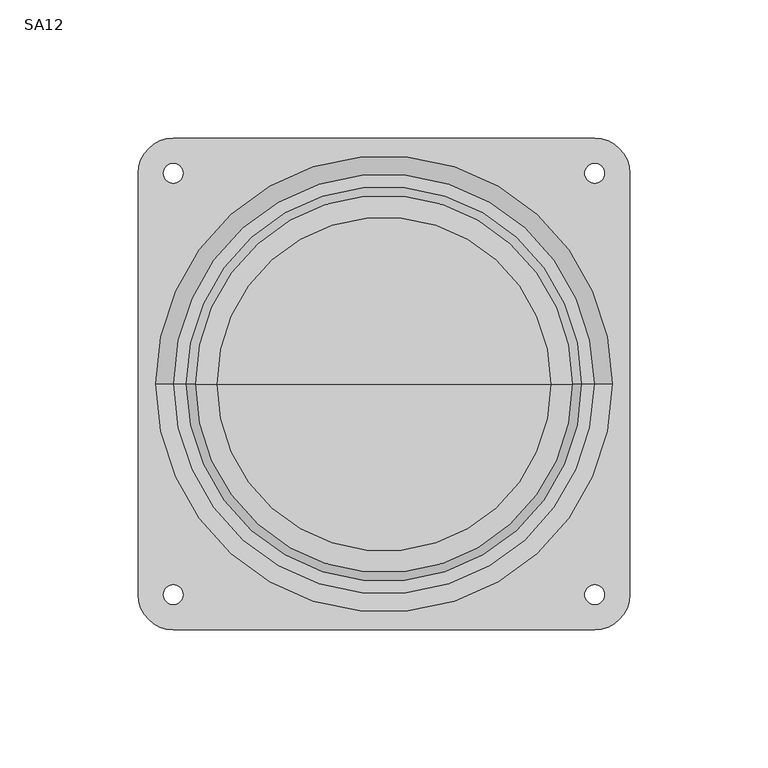
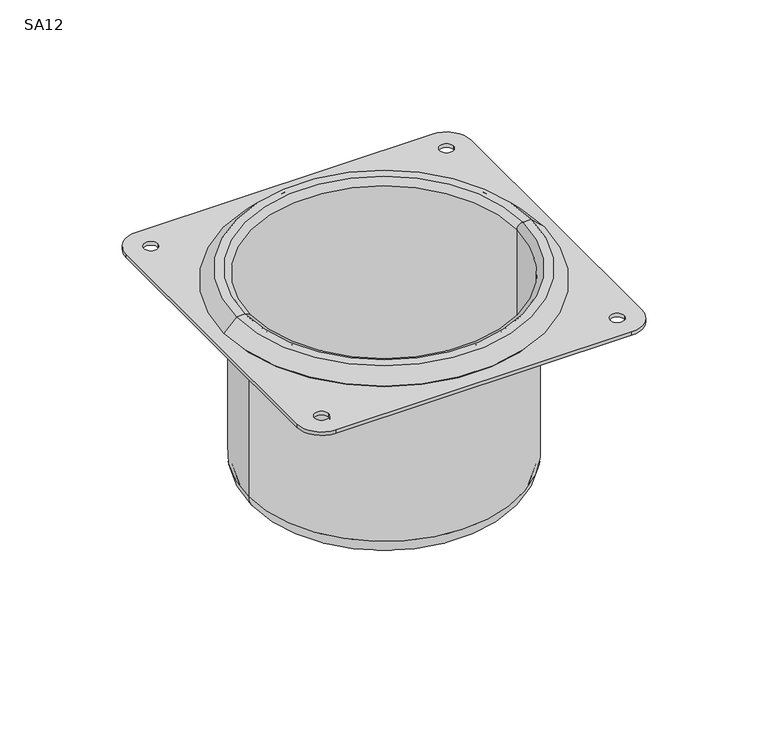
"""IFC4 building model written with IfcOpenShell, lengths in millimetres: proxy geometry, Security_Accessories-Bradley-SA12 : SA12."""

from ifc_helpers import new_model, si_unit, point, frame, frame_2d, origin, origin_with_axes, origin_2d, place, context, project, spatial, polyline, circle_curve, ellipse_curve, trimmed, segment, composite_curve, outline, extrude, source, transform, mapped, element, save
from ifc_brep_helpers import plane_surface, cylinder_surface, revolved_surface, advanced_brep


def sa12_a1c1abd2(model_context):
    return source(origin(), model_context, "Body", "SolidModel", [
        extrude(outline(composite_curve([segment(trimmed(circle_curve(frame_2d((-76.2, 76.2)), 12.7), [point((-88.9, 76.2))], [point((-76.2, 88.9))], False, "CARTESIAN"), True, "CONTINUOUS"), segment(polyline([(-76.2, 88.9), (76.2, 88.9)]), True, "CONTINUOUS"), segment(trimmed(circle_curve(frame_2d((76.2, 76.2)), 12.7), [point((76.2, 88.9))], [point((88.9, 76.2))], False, "CARTESIAN"), True, "CONTINUOUS"), segment(polyline([(88.9, 76.2), (88.9, -76.2)]), True, "CONTINUOUS"), segment(trimmed(circle_curve(frame_2d((76.2, -76.2)), 12.7), [point((88.9, -76.2))], [point((76.2, -88.9))], False, "CARTESIAN"), True, "CONTINUOUS"), segment(polyline([(76.2, -88.9), (-76.2, -88.9)]), True, "CONTINUOUS"), segment(trimmed(circle_curve(frame_2d((-76.2, -76.2)), 12.7), [point((-76.2, -88.9))], [point((-88.9, -76.2))], False, "CARTESIAN"), True, "CONTINUOUS"), segment(polyline([(-88.9, -76.2), (-88.9, 76.2)]), True, "CONTINUOUS")], self_intersect=False), holes=[composite_curve([segment(trimmed(circle_curve(frame_2d((-76.2, 76.2)), 3.571875), [point((-79.771875, 76.2))], [point((-72.628125, 76.2))], True, "CARTESIAN"), True, "CONTINUOUS"), segment(trimmed(circle_curve(frame_2d((-76.2, 76.2)), 3.571875), [point((-72.628125, 76.2))], [point((-79.771875, 76.2))], True, "CARTESIAN"), True, "CONTINUOUS")], self_intersect=False), composite_curve([segment(trimmed(circle_curve(frame_2d((-76.2, -76.2)), 3.571875), [point((-79.771875, -76.2))], [point((-72.628125, -76.2))], True, "CARTESIAN"), True, "CONTINUOUS"), segment(trimmed(circle_curve(frame_2d((-76.2, -76.2)), 3.571875), [point((-72.628125, -76.2))], [point((-79.771875, -76.2))], True, "CARTESIAN"), True, "CONTINUOUS")], self_intersect=False), composite_curve([segment(trimmed(circle_curve(frame_2d((76.2, -76.2)), 3.571875), [point((72.628125, -76.2))], [point((79.771875, -76.2))], True, "CARTESIAN"), True, "CONTINUOUS"), segment(trimmed(circle_curve(frame_2d((76.2, -76.2)), 3.571875), [point((79.771875, -76.2))], [point((72.628125, -76.2))], True, "CARTESIAN"), True, "CONTINUOUS")], self_intersect=False), composite_curve([segment(trimmed(circle_curve(frame_2d((76.2, 76.2)), 3.571875), [point((72.628125, 76.2))], [point((79.771875, 76.2))], True, "CARTESIAN"), True, "CONTINUOUS"), segment(trimmed(circle_curve(frame_2d((76.2, 76.2)), 3.571875), [point((79.771875, 76.2))], [point((72.628125, 76.2))], True, "CARTESIAN"), True, "CONTINUOUS")], self_intersect=False), composite_curve([segment(trimmed(circle_curve(origin_2d(), 81.4723693), [point((-81.4723693, 0.0))], [point((81.4723693, 0.0))], True, "CARTESIAN"), True, "CONTINUOUS"), segment(trimmed(circle_curve(origin_2d(), 81.4723693), [point((81.4723693, 0.0))], [point((-81.4723693, 0.0))], True, "CARTESIAN"), True, "CONTINUOUS")], self_intersect=False)]), origin_with_axes(), (0.0, 0.0, 1.0), 1.905),
        advanced_brep(
        [(68.326, 0.0, 6.4135), (-68.326, 0.0, 6.4135), (-68.326, 0.0, -90.551), (68.326, 0.0, -90.551), (71.4375, 0.0, 9.525), (-71.4375, 0.0, 9.525), (76.0076307, 0.0, 9.525), (-76.0076307, 0.0, 9.525), (82.55, 0.0, 2.9826307), (-82.55, 0.0, 2.9826307), (81.4723693, 0.0, 1.905), (-81.4723693, 0.0, 1.905), (75.3763693, 0.0, 8.001), (-75.3763693, 0.0, 8.001), (71.4375, 0.0, 8.001), (-71.4375, 0.0, 8.001), (69.85, 0.0, 6.4135), (-69.85, 0.0, 6.4135), (69.85, 0.0, -90.551), (-69.85, 0.0, -90.551), (60.3885, 0.0, -100.0125), (-60.3885, 0.0, -100.0125), (0.0, 0.0, -100.0125), (60.3885, 0.0, -98.4885), (-60.3885, 0.0, -98.4885), (0.0, 0.0, -98.4885)],
        [
            (0, 1, circle_curve(frame((0.0, 0.0, 6.4135), z_axis=(0.0, 0.0, 1.0), x_axis=(-1.0, 0.0, 0.0)), 68.326)),
            (1, 2),
            (2, 3, circle_curve(frame((0.0, 0.0, -90.551), z_axis=(0.0, 0.0, -1.0), x_axis=(-1.0, 0.0, 0.0)), 68.326)),
            (3, 0),
            (1, 0, circle_curve(frame((0.0, 0.0, 6.4135), z_axis=(0.0, 0.0, 1.0), x_axis=(-1.0, 0.0, 0.0)), 68.326)),
            (3, 2, circle_curve(frame((0.0, 0.0, -90.551), z_axis=(0.0, 0.0, -1.0), x_axis=(-1.0, 0.0, 0.0)), 68.326)),
            (4, 5, circle_curve(frame((0.0, 0.0, 9.525), z_axis=(0.0, 0.0, 1.0), x_axis=(-1.0, 0.0, 0.0)), 71.4375)),
            (5, 1, circle_curve(frame((-71.4375, 0.0, 6.4135), z_axis=(0.0, 1.0, 0.0), x_axis=(1.0, 0.0, 0.0)), 3.1115)),
            (0, 4, circle_curve(frame((71.4375, 0.0, 6.4135), z_axis=(0.0, 1.0, 0.0), x_axis=(-1.0, 0.0, 0.0)), 3.1115)),
            (5, 4, circle_curve(frame((0.0, 0.0, 9.525), z_axis=(0.0, 0.0, 1.0), x_axis=(-1.0, 0.0, 0.0)), 71.4375)),
            (6, 7, circle_curve(frame((0.0, 0.0, 9.525), z_axis=(0.0, 0.0, 1.0), x_axis=(-1.0, 0.0, 0.0)), 76.0076307)),
            (7, 5),
            (4, 6),
            (7, 6, circle_curve(frame((0.0, 0.0, 9.525), z_axis=(0.0, 0.0, 1.0), x_axis=(-1.0, 0.0, 0.0)), 76.0076307)),
            (8, 9, circle_curve(frame((0.0, 0.0, 2.9826307), z_axis=(0.0, 0.0, 1.0), x_axis=(-1.0, 0.0, 0.0)), 82.55)),
            (9, 7),
            (6, 8),
            (9, 8, circle_curve(frame((0.0, 0.0, 2.9826307), z_axis=(0.0, 0.0, 1.0), x_axis=(-1.0, 0.0, 0.0)), 82.55)),
            (10, 11, circle_curve(frame((0.0, 0.0, 1.905), z_axis=(0.0, 0.0, 1.0), x_axis=(-1.0, 0.0, 0.0)), 81.4723693)),
            (11, 9),
            (8, 10),
            (11, 10, circle_curve(frame((0.0, 0.0, 1.905), z_axis=(0.0, 0.0, 1.0), x_axis=(-1.0, 0.0, 0.0)), 81.4723693)),
            (12, 13, circle_curve(frame((0.0, 0.0, 8.001), z_axis=(0.0, 0.0, 1.0), x_axis=(-1.0, 0.0, 0.0)), 75.3763693)),
            (13, 11),
            (10, 12),
            (13, 12, circle_curve(frame((0.0, 0.0, 8.001), z_axis=(0.0, 0.0, 1.0), x_axis=(-1.0, 0.0, 0.0)), 75.3763693)),
            (14, 15, circle_curve(frame((0.0, 0.0, 8.001), z_axis=(0.0, 0.0, 1.0), x_axis=(-1.0, 0.0, 0.0)), 71.4375)),
            (15, 13),
            (12, 14),
            (15, 14, circle_curve(frame((0.0, 0.0, 8.001), z_axis=(0.0, 0.0, 1.0), x_axis=(-1.0, 0.0, 0.0)), 71.4375)),
            (16, 17, circle_curve(frame((0.0, 0.0, 6.4135), z_axis=(0.0, 0.0, 1.0), x_axis=(-1.0, 0.0, 0.0)), 69.85)),
            (17, 15, circle_curve(frame((-71.4375, 0.0, 6.4135), z_axis=(0.0, -1.0, 0.0), x_axis=(1.0, 0.0, 0.0)), 1.5875)),
            (14, 16, circle_curve(frame((71.4375, 0.0, 6.4135), z_axis=(0.0, -1.0, 0.0), x_axis=(-1.0, 0.0, 0.0)), 1.5875)),
            (17, 16, circle_curve(frame((0.0, 0.0, 6.4135), z_axis=(0.0, 0.0, 1.0), x_axis=(-1.0, 0.0, 0.0)), 69.85)),
            (18, 19, circle_curve(frame((0.0, 0.0, -90.551), z_axis=(0.0, 0.0, 1.0), x_axis=(-1.0, 0.0, 0.0)), 69.85)),
            (19, 17),
            (16, 18),
            (19, 18, circle_curve(frame((0.0, 0.0, -90.551), z_axis=(0.0, 0.0, 1.0), x_axis=(-1.0, 0.0, 0.0)), 69.85)),
            (20, 21, circle_curve(frame((0.0, 0.0, -100.0125), z_axis=(0.0, 0.0, 1.0), x_axis=(-1.0, 0.0, 0.0)), 60.3885)),
            (21, 19, circle_curve(frame((-60.3885, 0.0, -90.551), z_axis=(0.0, 1.0, 0.0), x_axis=(1.0, 0.0, 0.0)), 9.4615)),
            (18, 20, circle_curve(frame((60.3885, 0.0, -90.551), z_axis=(0.0, 1.0, 0.0), x_axis=(-1.0, 0.0, 0.0)), 9.4615)),
            (21, 20, circle_curve(frame((0.0, 0.0, -100.0125), z_axis=(0.0, 0.0, 1.0), x_axis=(-1.0, 0.0, 0.0)), 60.3885)),
            (22, 21),
            (20, 22),
            (23, 24, circle_curve(frame((0.0, 0.0, -98.4885), z_axis=(0.0, 0.0, 1.0), x_axis=(-1.0, 0.0, 0.0)), 60.3885)),
            (24, 25),
            (25, 23),
            (24, 23, circle_curve(frame((0.0, 0.0, -98.4885), z_axis=(0.0, 0.0, 1.0), x_axis=(-1.0, 0.0, 0.0)), 60.3885)),
            (2, 24, circle_curve(frame((-60.3885, 0.0, -90.551), z_axis=(0.0, -1.0, 0.0), x_axis=(1.0, 0.0, 0.0)), 7.9375)),
            (23, 3, circle_curve(frame((60.3885, 0.0, -90.551), z_axis=(0.0, -1.0, 0.0), x_axis=(-1.0, 0.0, 0.0)), 7.9375)),
        ],
        [
            revolved_surface(polyline([(-68.326, 0.0, -90.551), (-68.326, 0.0, 6.413499999999999)]), (0.0, 0.0, -119.0625), (0.0, 0.0, -1.0)),
            revolved_surface(trimmed(ellipse_curve(frame((-71.4375, 0.0, 6.4135), z_axis=(0.0, -1.0, 0.0), x_axis=(1.0, 0.0, 0.0)), 3.1115, 3.1115), [point((-68.326, 0.0, 6.4135))], [point((-71.4375, 0.0, 9.525))], True, "CARTESIAN"), (0.0, 0.0, -119.0625), (0.0, 0.0, -1.0)),
            plane_surface(frame((0.0, 0.0, 9.525), z_axis=(0.0, 0.0, 1.0), x_axis=(-1.0, 0.0, 0.0))),
            revolved_surface(polyline([(-76.0076307, 0.0, 9.525), (-82.55, 0.0, 2.9826307)]), (0.0, 0.0, -119.0625), (0.0, 0.0, -1.0)),
            revolved_surface(polyline([(-82.55, 0.0, 2.9826307), (-81.4723693, 0.0, 1.905)]), (0.0, 0.0, -119.0625), (0.0, 0.0, -1.0)),
            revolved_surface(polyline([(-81.4723693, 0.0, 1.905), (-75.3763693, 0.0, 8.001)]), (0.0, 0.0, -119.0625), (0.0, 0.0, -1.0)),
            plane_surface(frame((0.0, 0.0, 8.001), z_axis=(0.0, 0.0, -1.0), x_axis=(-1.0, 0.0, 0.0))),
            revolved_surface(trimmed(ellipse_curve(frame((-71.4375, 0.0, 6.4135), z_axis=(0.0, 1.0, 0.0), x_axis=(1.0, 0.0, 0.0)), 1.5875, 1.5875), [point((-71.4375, 0.0, 8.001))], [point((-69.85, 0.0, 6.4135))], True, "CARTESIAN"), (0.0, 0.0, -119.0625), (0.0, 0.0, -1.0)),
            cylinder_surface(frame((0.0, 0.0, -119.0625), z_axis=(0.0, 0.0, -1.0), x_axis=(-1.0, 0.0, 0.0)), 69.85),
            revolved_surface(trimmed(ellipse_curve(frame((-60.3885, 0.0, -90.551), z_axis=(0.0, -1.0, 0.0), x_axis=(1.0, 0.0, 0.0)), 9.4615, 9.4615), [point((-69.85, 0.0, -90.551))], [point((-60.3885, 0.0, -100.0125))], True, "CARTESIAN"), (0.0, 0.0, -119.0625), (0.0, 0.0, -1.0)),
            plane_surface(frame((0.0, 0.0, -100.0125), z_axis=(0.0, 0.0, -1.0), x_axis=(-1.0, 0.0, 0.0))),
            plane_surface(frame((0.0, 0.0, -98.4885), z_axis=(0.0, 0.0, 1.0), x_axis=(-1.0, 0.0, 0.0))),
            revolved_surface(trimmed(ellipse_curve(frame((-60.3885, 0.0, -90.551), z_axis=(0.0, 1.0, 0.0), x_axis=(1.0, 0.0, 0.0)), 7.9375, 7.9375), [point((-60.3885, 0.0, -98.4885))], [point((-68.326, 0.0, -90.551))], True, "CARTESIAN"), (0.0, 0.0, -119.0625), (0.0, 0.0, -1.0)),
        ],
        [
            (0, [[1, 2, 3, 4]]),
            (0, [[5, -4, 6, -2]]),
            (1, [[7, 8, -1, 9]]),
            (1, [[10, -9, -5, -8]]),
            (2, [[11, 12, -7, 13]]),
            (2, [[14, -13, -10, -12]]),
            (3, [[15, 16, -11, 17]]),
            (3, [[18, -17, -14, -16]]),
            (4, [[19, 20, -15, 21]]),
            (4, [[22, -21, -18, -20]]),
            (5, [[23, 24, -19, 25]]),
            (5, [[26, -25, -22, -24]]),
            (6, [[27, 28, -23, 29]]),
            (6, [[30, -29, -26, -28]]),
            (7, [[31, 32, -27, 33]]),
            (7, [[34, -33, -30, -32]]),
            (8, [[35, 36, -31, 37]]),
            (8, [[38, -37, -34, -36]]),
            (9, [[39, 40, -35, 41]]),
            (9, [[42, -41, -38, -40]]),
            (10, [[43, -39, 44]]),
            (10, [[-44, -42, -43]]),
            (11, [[45, 46, 47]]),
            (11, [[48, -47, -46]]),
            (12, [[-3, 49, -45, 50]]),
            (12, [[-6, -50, -48, -49]]),
        ],
    ),
    ])


if __name__ == "__main__":
    model = new_model("IFC4")
    model_context = context("Model", 3, world=origin())
    ifc_project = project(units=[si_unit("LENGTHUNIT", "METRE", prefix="MILLI")], contexts=[model_context])
    site = spatial("IfcSite", under=ifc_project)
    building = spatial("IfcBuilding", under=site)
    placement = place(None, origin())
    sa12_shape = sa12_a1c1abd2(model_context)
    element("IfcBuildingElementProxy", 1, Name="Security_Accessories-Bradley-SA12 : SA12", ObjectType="Security_Accessories-Bradley-SA12 : SA12", at=placement, inside=building, context=model_context, shape_type="MappedRepresentation", body=[
        mapped(sa12_shape, transform((0.0, 0.0, 0.0), x_axis=(1.0, 0.0, 0.0), y_axis=(0.0, 1.0, 0.0), z_axis=(0.0, 0.0, 1.0))),
    ])
    save(model, "model.ifc")

# Revit data of these elements
# Type "Security_Accessories-Bradley-SA12 : SA12"
#   Warranty Information = "Complete Unit - One Year"
#   Version = "1.0"
#   URL = "http://www.bradleycorp.com/"
#   OmniClass Title = "Toilet Tissue Dispensers"
#   OmniClass Code = "23.21.43.15.31"
#   Modeling Code = ""
#   Model = "SA12"
#   MasterFormat Title = "Security Toilet Accessories"
#   MasterFormat Number = "10 28 13.53"
#   Manufacturer = "Bradley Corporation"
#   Industry Standards = ""
#   Fire Rating = ""
#   Description = "Security Toilet Tissue Roll Holder"
#   Copyright = "This Model Data is Property of Bradley Corporation"
#   Buy American Act = "Yes"
#   Assembly Code = "C1030200"
#   ADA Compliant = "Yes"
#   Width = 177.8 mm
#   Height = 177.8 mm
#   Default Elevation = 1219.2 mm
#   Material = Metal - Bradley Corp - Stainless Steel - Satin
# Element 1 (IfcBuildingElementProxy, "Security_Accessories-Bradley-SA12 : SA12")
#   Materials on its faces: "Metal - Bradley Corp - Stainless Steel - Satin"
# Materials
#   "Metal - Bradley Corp - Stainless Steel - Satin": class "Metal", colour RGB 189 187 185, transparency 0, Manufacturer = "Bradley Corporation", URL = "www.bradleycorp.com", Description = "Stainless Steel - Satin Finish", Cost = 0
